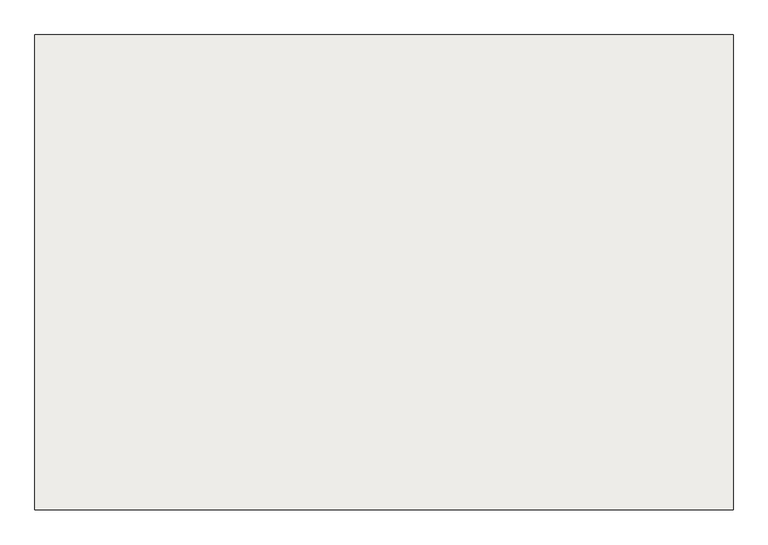
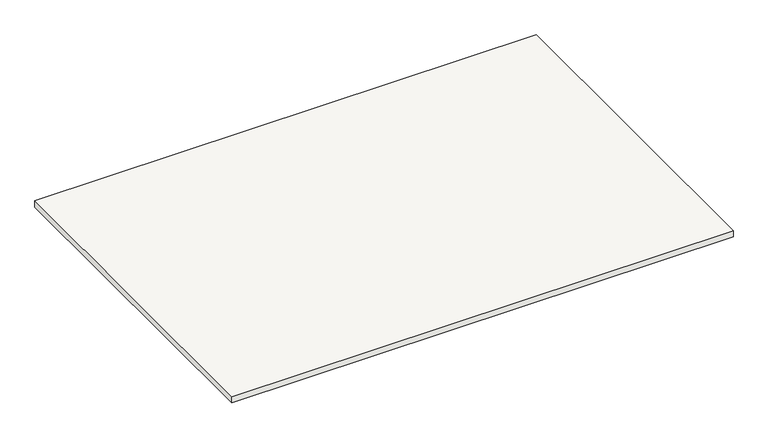
"""IFC4 building model written with IfcOpenShell, lengths in millimetres: slab geometry."""

from ifc_helpers import new_model, si_unit, frame, origin, place, context, project, spatial, polyline, outline, extrude, source, transform, mapped, element, save


def slab_6da8d7b7(model_context):
    return source(origin(), model_context, "Body", "SweptSolid", [
        extrude(outline(polyline([(3809.5374538, 37424.5208589), (3809.5374538, 37232.6086665), (3809.5374538, 36032.6086665), (0.0, 36032.6086665), (0.0, 38624.5208589), (3809.5374538, 38624.5208589), (3809.5374538, 37424.5208589)])), frame((0.0, 0.0, 2549.9720055), z_axis=(0.0, 0.0, 1.0), x_axis=(1.0, 0.0, 0.0)), (0.0, 0.0, 1.0), 50.0),
    ])


if __name__ == "__main__":
    model = new_model("IFC4")
    model_context = context("Model", 3, world=origin())
    ifc_project = project(units=[si_unit("LENGTHUNIT", "METRE", prefix="MILLI")], contexts=[model_context])
    site = spatial("IfcSite", under=ifc_project)
    building = spatial("IfcBuilding", under=site)
    placement = place(None, origin())
    slab_shape = slab_6da8d7b7(model_context)
    element("IfcSlab", 1, at=placement, inside=building, context=model_context, shape_type="MappedRepresentation", body=[
        mapped(slab_shape, transform((0.0, 0.0, 0.0), x_axis=(1.0, 0.0, 0.0), y_axis=(0.0, 1.0, 0.0), z_axis=(0.0, 0.0, 1.0))),
    ])
    save(model, "model.ifc")
